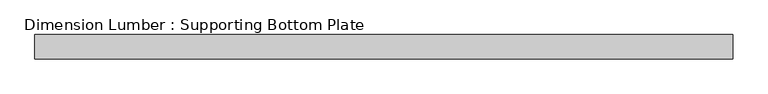
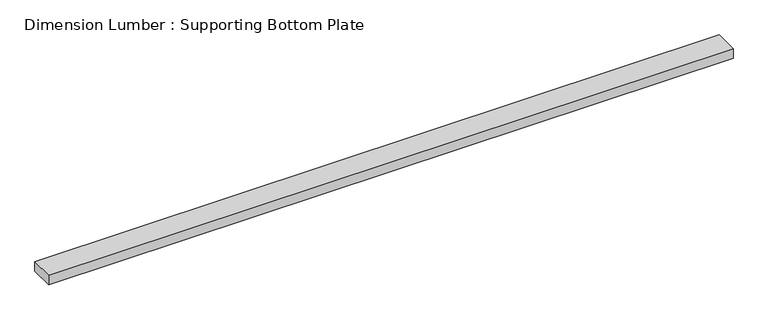
"""IFC4 building model written with IfcOpenShell, lengths in millimetres: beam geometry, Dimension Lumber : Supporting Bottom Plate."""

from ifc_helpers import new_model, si_unit, frame, origin, place, context, project, spatial, polyline, outline, extrude, source, transform, mapped, element, save


def dimension_lumber_supporting_bottom_plate_9bff56d6(model_context):
    return source(origin(), model_context, "Body", "SweptSolid", [
        extrude(outline(polyline([(-1544.0421875, 44.45), (-1544.0421875, -44.45), (-4097.9328125, -44.45), (-4097.9328125, 44.45), (-1544.0421875, 44.45)])), frame((0.0, 0.0, -19.05), z_axis=(0.0, 0.0, 1.0), x_axis=(1.0, 0.0, 0.0)), (0.0, 0.0, 1.0), 38.1),
    ])


if __name__ == "__main__":
    model = new_model("IFC4")
    model_context = context("Model", 3, world=origin())
    ifc_project = project(units=[si_unit("LENGTHUNIT", "METRE", prefix="MILLI")], contexts=[model_context])
    site = spatial("IfcSite", under=ifc_project)
    building = spatial("IfcBuilding", under=site)
    placement = place(None, origin())
    dimension_lumber_supporting_bottom_plate_shape = dimension_lumber_supporting_bottom_plate_9bff56d6(model_context)
    element("IfcBeam", 1, ObjectType="Dimension Lumber : Supporting Bottom Plate", at=placement, inside=building, context=model_context, shape_type="MappedRepresentation", body=[
        mapped(dimension_lumber_supporting_bottom_plate_shape, transform((0.0, 0.0, 0.0), x_axis=(1.0, 0.0, 0.0), y_axis=(0.0, 1.0, 0.0), z_axis=(0.0, 0.0, 1.0))),
    ])
    save(model, "model.ifc")

# Revit data of these elements
# Type "Dimension Lumber : Supporting Bottom Plate"
#   Assembly Code = "B10"
#   A = 0.0364583 SF
#   Length [instance default] = 5' - 0"
#   b = 0' - 3 1/2"
#   d = 0' - 1 1/2"
#   Structural Material [instance default] = Softwood, Lumber
# Element 1 (IfcBeam, "Dimension Lumber : Supporting Bottom Plate")
#   Structural Material = Douglas Fir #2
#   Materials on its faces: "Douglas Fir #2"
# Materials
#   "Softwood, Lumber": class "Wood", colour RGB 223 192 134, transparency 0, Description = "Pinus Echinata", Cost = 0
#   "Douglas Fir #2": class "Wood", colour RGB 223 192 134, transparency 0, Description = "Pinus Echinata", Cost = 0
